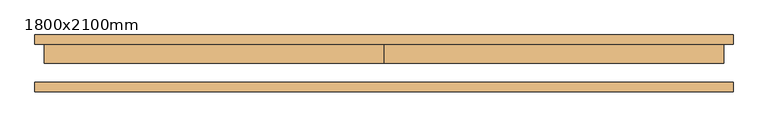
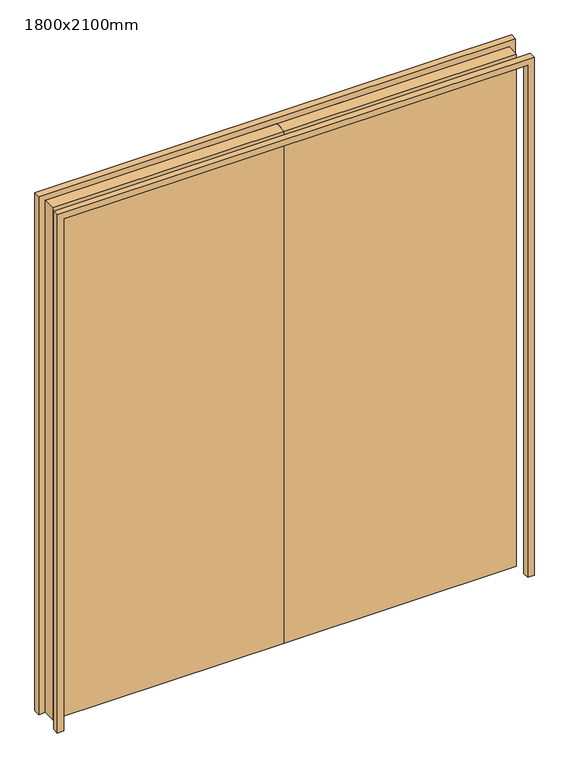
"""IFC4 building model written with IfcOpenShell, lengths in millimetres: door geometry, WWm-DoubleSolid-Flush : 1800x2100mm."""

from ifc_helpers import new_model, si_unit, frame, origin, origin_with_axes, place, context, project, spatial, polyline, outline, extrude, source, transform, mapped, element, save


def door_1800x2100mm_2eb4d894(model_context):
    return source(origin(), model_context, "Body", "SweptSolid", [
        extrude(outline(polyline([(0.0, 50.0), (900.0, 50.0), (900.0, 0.0), (0.0, 0.0), (0.0, 50.0)])), origin_with_axes(), (0.0, 0.0, 1.0), 2100.0),
        extrude(outline(polyline([(-900.0, 50.0), (0.0, 50.0), (0.0, 0.0), (-900.0, 0.0), (-900.0, 50.0)])), origin_with_axes(), (0.0, 0.0, 1.0), 2100.0),
        extrude(outline(polyline([(2100.0, -900.0), (2100.0, 900.0), (0.0, 900.0), (0.0, 925.0), (2125.0, 925.0), (2125.0, -925.0), (0.0, -925.0), (0.0, -900.0), (2100.0, -900.0)])), frame((0.0, -75.0, 0.0), z_axis=(0.0, 1.0, 0.0), x_axis=(0.0, 0.0, 1.0)), (0.0, 0.0, 1.0), 25.0),
        extrude(outline(polyline([(2100.0, -900.0), (2100.0, 900.0), (0.0, 900.0), (0.0, 925.0), (2125.0, 925.0), (2125.0, -925.0), (0.0, -925.0), (0.0, -900.0), (2100.0, -900.0)])), frame((0.0, 50.0, 0.0), z_axis=(0.0, 1.0, 0.0), x_axis=(0.0, 0.0, 1.0)), (0.0, 0.0, 1.0), 25.0),
    ])


if __name__ == "__main__":
    model = new_model("IFC4")
    model_context = context("Model", 3, world=origin())
    ifc_project = project(units=[si_unit("LENGTHUNIT", "METRE", prefix="MILLI")], contexts=[model_context])
    site = spatial("IfcSite", under=ifc_project)
    building = spatial("IfcBuilding", under=site)
    placement = place(None, origin())
    door_1800x2100mm_shape = door_1800x2100mm_2eb4d894(model_context)
    element("IfcDoor", 1, ObjectType="WWm-DoubleSolid-Flush : 1800x2100mm", at=placement, inside=building, context=model_context, shape_type="MappedRepresentation", body=[
        mapped(door_1800x2100mm_shape, transform((0.0, 0.0, 0.0), x_axis=(1.0, 0.0, 0.0), y_axis=(0.0, 1.0, 0.0), z_axis=(0.0, 0.0, 1.0))),
    ])
    save(model, "model.ifc")

# Revit data of these elements
# Type "WWm-DoubleSolid-Flush : 1800x2100mm"
#   Type Mark = "EX1-44"
#   Construction Type Id = "MDOOR"
#   Assembly Code = "C1020"
#   Analytic Construction = "Metal"
#   Thickness = 50 mm
#   Thermal Resistance (R) = 0.270117 (m²·K)/W
#   Heat Transfer Coefficient (U) = 3.7021 W/(m²·K)
#   Height = 2100 mm
#   Trim Projection Ext = 25 mm
#   Trim Projection Int = 25 mm
#   Trim Width = 25 mm
#   Width = 1800 mm
#   Not 90 Degree [instance default] = no
#   90 Degree [instance default] = yes
#   Door Material = WW-EC-RGB-White
#   Frame Material = WW-EC-RGB-White
#   Visual Light Transmittance = 0
#   Solar Heat Gain Coefficient = 0
#   Function = (empty or 0)
#   Wall Closure = (empty or 0)
# Element 1 (IfcDoor, "WWm-DoubleSolid-Flush : 1800x2100mm")
#   Materials on its faces: "WW-EC-RGB-White"
# Materials
#   "WW-EC-RGB-White": class "Generic", colour RGB 255 255 255, transparency 0, Comments = "If region requests off-white, swith asset color to RGB 231-228-220", Description = "Generic Color", Cost = 0
